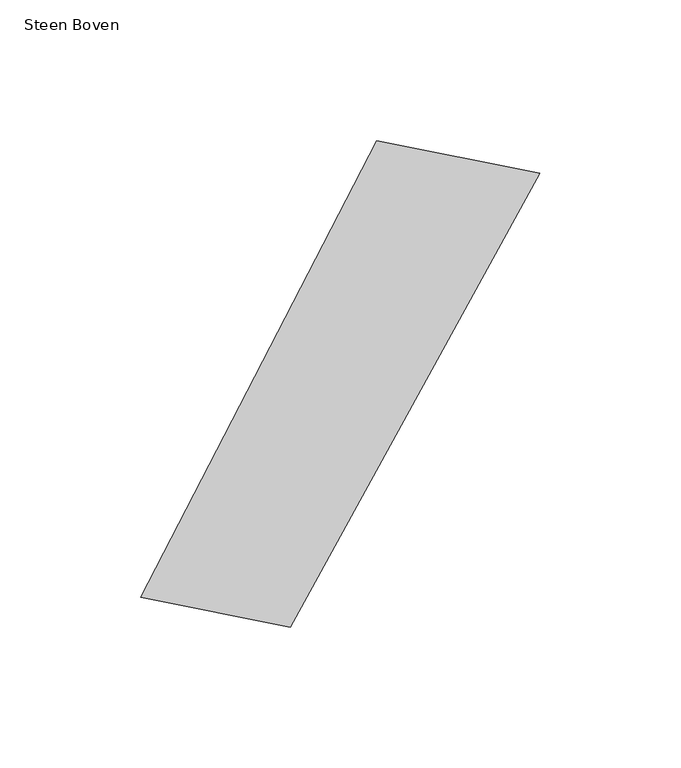
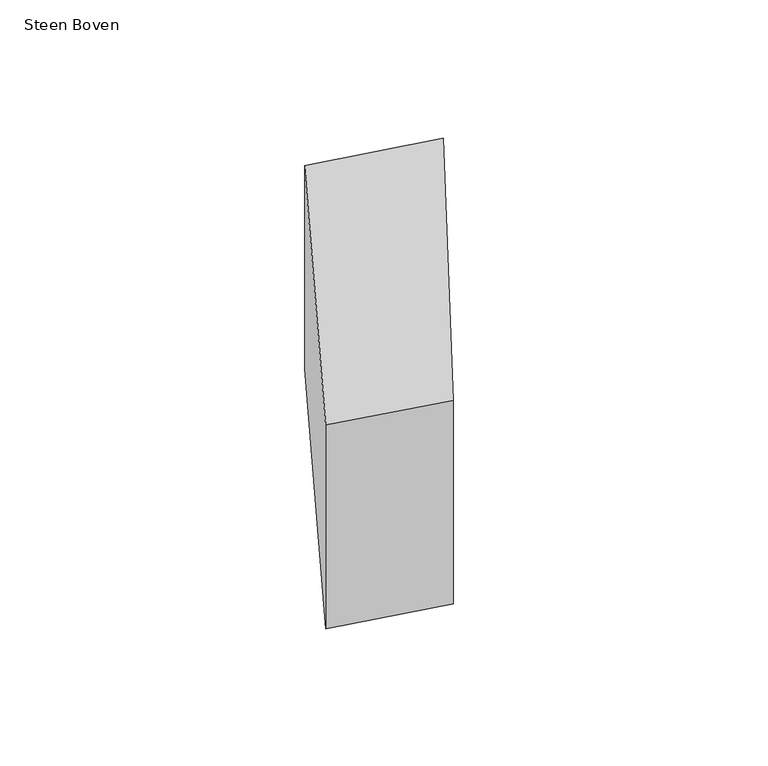
"""IFC4 building model written with IfcOpenShell, lengths in millimetres: proxy geometry, 00_GMA_steen_versie_4 : Steen Boven."""

from ifc_helpers import new_model, si_unit, origin, origin_with_axes, place, context, project, spatial, polyline, outline, extrude, source, transform, mapped, element, save


def steen_boven_eabcd001(model_context):
    return source(origin(), model_context, "Body", "SweptSolid", [
        extrude(outline(polyline([(146.1086958, 152.321622), (57.5952589, -8.8049317), (4.5075261, 1.71935), (88.2622432, 163.7549131), (146.1086958, 152.321622)])), origin_with_axes(), (0.0, 0.0, 1.0), 100.0),
    ])


if __name__ == "__main__":
    model = new_model("IFC4")
    model_context = context("Model", 3, world=origin())
    ifc_project = project(units=[si_unit("LENGTHUNIT", "METRE", prefix="MILLI")], contexts=[model_context])
    site = spatial("IfcSite", under=ifc_project)
    building = spatial("IfcBuilding", under=site)
    placement = place(None, origin())
    steen_boven_shape = steen_boven_eabcd001(model_context)
    element("IfcBuildingElementProxy", 1, Name="00_GMA_steen_versie_4 : Steen Boven", ObjectType="00_GMA_steen_versie_4 : Steen Boven", at=placement, inside=building, context=model_context, shape_type="MappedRepresentation", body=[
        mapped(steen_boven_shape, transform((0.0, 0.0, 0.0), x_axis=(1.0, 0.0, 0.0), y_axis=(0.0, 1.0, 0.0), z_axis=(0.0, 0.0, 1.0))),
    ])
    save(model, "model.ifc")

# Revit data of these elements
# Type "00_GMA_steen_versie_4 : Steen Boven"
#   StootVoegHalfBoven [instance default] = 5 mm
#   StootVoegHalf [instance default] = 5 mm
#   StootVoegBreedteOnder = 10 mm
#   StootVoegBreedteBoven = 10 mm
#   Steendikte = 100 mm
#   LintVoegOnderHalf = 5 mm
#   LintVoegOnder = 10 mm
#   LintVoegBovenHalf = 0 mm
#   LintVoegBoven = 0 mm
#   materiaal = none
#   MateriaalVoeg = none
#   Default Elevation = 0
